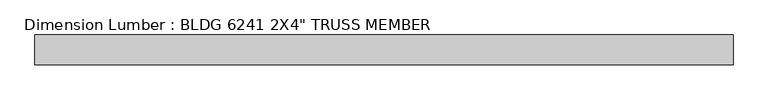
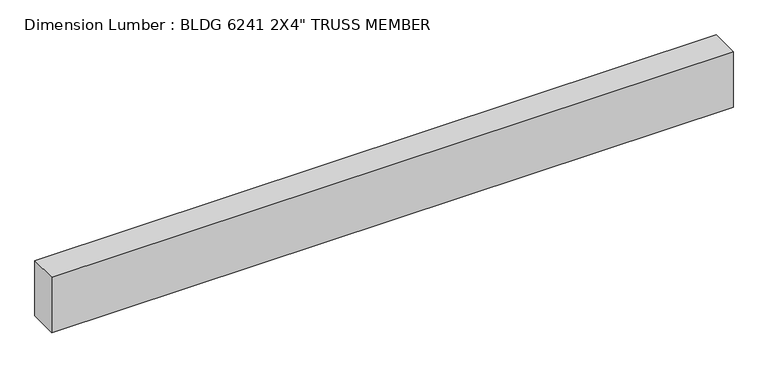
"""IFC4 building model written with IfcOpenShell, lengths in millimetres: beam geometry."""

import ifcopenshell
import ifcopenshell.guid

model = None  # the IFC model being written
_history = None  # IfcOwnerHistory: only IFC2X3 demands one
_inside = {}  # id of a spatial element -> (the spatial element, [elements in it])
_under = {}  # id of a project, library or spatial element -> (it, [spatial elements below it])
_declared = {}  # id of a project -> (the project, [libraries it declares])
_typed = {}  # id of a type object -> (the type object, [elements of that type])
_made_of = {}  # id of a material, layer set ... -> (it, [elements and type objects made of it])


def new_model(schema):
    """Start an empty IFC model of exactly this schema.

    Asked for "IFC4X3", IfcOpenShell would pick the latest addendum, in which some entities
    have other attributes; the version numbers below select the first issue.
    IFC2X3 requires an IfcOwnerHistory on every rooted entity: one is made here for all.
    """
    global model, _history
    if schema == "IFC4X3":
        model = ifcopenshell.file(schema_version=(4, 3, 0, 0))
    else:
        model = ifcopenshell.file(schema=schema)
    _inside.clear()
    _under.clear()
    _declared.clear()
    _typed.clear()
    _made_of.clear()
    _history = None
    if model.schema == "IFC2X3":
        org = make("IfcOrganization", Name="unknown")
        user = make(
            "IfcPersonAndOrganization",
            ThePerson=make("IfcPerson", FamilyName="unknown"),
            TheOrganization=org,
        )
        app = make(
            "IfcApplication",
            ApplicationDeveloper=org,
            Version="unknown",
            ApplicationFullName="unknown",
            ApplicationIdentifier="unknown",
        )
        _history = make(
            "IfcOwnerHistory",
            OwningUser=user,
            OwningApplication=app,
            ChangeAction="ADDED",
            CreationDate=0,
        )
    return model


def make(cls, **values):
    """One entity of the class cls with the attributes given. An attribute that is None is left unset."""
    return model.create_entity(
        cls, **{name: value for name, value in values.items() if value is not None}
    )


def rooted(cls, **values):
    """An entity with a GlobalId (a new one), such as an element, a storey or a relation."""
    return make(cls, GlobalId=ifcopenshell.guid.new(), OwnerHistory=_history, **values)


def si_unit(unit_type, name, prefix=None):
    """IfcSIUnit, for example si_unit("LENGTHUNIT", "METRE", prefix="MILLI")."""
    return make("IfcSIUnit", UnitType=unit_type, Prefix=prefix, Name=name)


def assignment(units):
    """IfcUnitAssignment: the units of a project."""
    return None if units is None else make("IfcUnitAssignment", Units=units)


def point(xyz):
    """IfcCartesianPoint."""
    return None if xyz is None else make("IfcCartesianPoint", Coordinates=xyz)


def direction(xyz):
    """IfcDirection."""
    return None if xyz is None else make("IfcDirection", DirectionRatios=xyz)


def frame(location, z_axis=None, x_axis=None):
    """IfcAxis2Placement3D, a coordinate frame: its origin and axes. An axis left out is left unset."""
    return make(
        "IfcAxis2Placement3D",
        Location=point(location),
        Axis=direction(z_axis),
        RefDirection=direction(x_axis),
    )


def origin():
    """The frame at (0, 0, 0) with its axes left unset."""
    return frame((0.0, 0.0, 0.0))


def place(relative_to, where):
    """IfcLocalPlacement: puts the frame where relative to a parent placement (None: the world)."""
    return make(
        "IfcLocalPlacement", PlacementRelTo=relative_to, RelativePlacement=where
    )


def context(
    kind, dimensions, precision=None, world=None, true_north=None, identifier=None
):
    """IfcGeometricRepresentationContext, for example the 3D "Model" context."""
    return make(
        "IfcGeometricRepresentationContext",
        ContextIdentifier=identifier,
        ContextType=kind,
        CoordinateSpaceDimension=dimensions,
        Precision=precision,
        WorldCoordinateSystem=world,
        TrueNorth=true_north,
    )


def project(units=None, contexts=None):
    """IfcProject with its units and contexts."""
    return rooted(
        "IfcProject",
        Name="project",
        RepresentationContexts=contexts,
        UnitsInContext=assignment(units),
    )


def spatial(cls, under=None, at=None, **own):
    """A site, building, storey or space (cls), placed at a placement, below another one or the project."""
    s = rooted(cls, ObjectPlacement=at, **own)
    if under is not None:
        _under.setdefault(under.id(), (under, []))[1].append(s)
    return s


def polyline(points):
    """IfcPolyline through the points."""
    return make("IfcPolyline", Points=[point(p) for p in points])


def outline(outer, holes=None, kind="AREA"):
    """IfcArbitraryClosedProfileDef: a profile drawn as a closed curve; with holes, ...WithVoids."""
    if holes is None:
        return make("IfcArbitraryClosedProfileDef", ProfileType=kind, OuterCurve=outer)
    return make(
        "IfcArbitraryProfileDefWithVoids",
        ProfileType=kind,
        OuterCurve=outer,
        InnerCurves=holes,
    )


def extrude(swept, where, along, depth):
    """IfcExtrudedAreaSolid: the profile swept, set in the frame where, extruded along a direction by depth."""
    return make(
        "IfcExtrudedAreaSolid",
        SweptArea=swept,
        Position=where,
        ExtrudedDirection=direction(along),
        Depth=depth,
    )


def shape(context_of_items, identifier, shape_type, items):
    """IfcShapeRepresentation: the items that make up one representation, for example the "Body"."""
    return make(
        "IfcShapeRepresentation",
        ContextOfItems=context_of_items,
        RepresentationIdentifier=identifier,
        RepresentationType=shape_type,
        Items=items,
    )


def source(mapping_origin, context_of_items, identifier, shape_type, items):
    """IfcRepresentationMap: a shape defined once, which mapped items show again and again."""
    return make(
        "IfcRepresentationMap",
        MappingOrigin=mapping_origin,
        MappedRepresentation=shape(context_of_items, identifier, shape_type, items),
    )


def transform(
    local_origin,
    x_axis=None,
    y_axis=None,
    z_axis=None,
    scale=None,
    scale2=None,
    scale3=None,
    uniform=True,
):
    """IfcCartesianTransformationOperator3D, or its non-uniform kind. x_axis, y_axis, z_axis: its Axis1, 2, 3."""
    if uniform:
        return make(
            "IfcCartesianTransformationOperator3D",
            Axis1=direction(x_axis),
            Axis2=direction(y_axis),
            LocalOrigin=point(local_origin),
            Scale=scale,
            Axis3=direction(z_axis),
        )
    return make(
        "IfcCartesianTransformationOperator3DnonUniform",
        Axis1=direction(x_axis),
        Axis2=direction(y_axis),
        LocalOrigin=point(local_origin),
        Scale=scale,
        Axis3=direction(z_axis),
        Scale2=scale2,
        Scale3=scale3,
    )


def mapped(mapping_source, mapping_target):
    """IfcMappedItem: shows the shape of a source again, moved by a transform."""
    return make(
        "IfcMappedItem", MappingSource=mapping_source, MappingTarget=mapping_target
    )


def made_of(thing, what):
    """Note that an element or type object is made of a material, layer set ...; save() writes the relation."""
    if what is not None:
        _made_of.setdefault(what.id(), (what, []))[1].append(thing)
    return thing


def element(
    cls,
    number,
    at=None,
    inside=None,
    cuts=None,
    type_object=None,
    material=None,
    context=None,
    identifier="Body",
    shape_type=None,
    held_by="IfcProductDefinitionShape",
    body=None,
    shapes=None,
    **own,
):
    """One element of the class cls, such as IfcWall. Its Tag is "e" and its number.

    at: its placement. inside: the storey or other place that contains it. cuts: it is an
    opening in that element (IfcRelVoidsElement). A single representation is given by context,
    identifier, shape_type and body (its items); several are given by shapes. held_by: the class
    of the entity that holds the representations. save() writes the other relations.
    """
    e = rooted(cls, Tag="e%d" % number, ObjectPlacement=at, **own)
    if body is not None:
        shapes = [shape(context, identifier, shape_type, body)]
    if shapes is not None:
        e.Representation = make(held_by, Representations=shapes)
    if inside is not None:
        _inside.setdefault(inside.id(), (inside, []))[1].append(e)
    if cuts is not None:
        rooted(
            "IfcRelVoidsElement", RelatingBuildingElement=cuts, RelatedOpeningElement=e
        )
    if type_object is not None:
        _typed.setdefault(type_object.id(), (type_object, []))[1].append(e)
    return made_of(e, material)


def aggregate(whole, parts):
    """IfcRelAggregates: a whole, such as a stair, and the parts it consists of."""
    return rooted("IfcRelAggregates", RelatingObject=whole, RelatedObjects=parts)


def save(model, path):
    """Write the relations noted so far, then the file.

    IfcRelAggregates (storeys below a building ...), IfcRelContainedInSpatialStructure (elements
    in a storey), IfcRelDefinesByType, IfcRelAssociatesMaterial and IfcRelDeclares: one each for
    every whole, place, type object, material and project.
    """
    for whole, parts in _under.values():
        aggregate(whole, parts)
    for where, things in _inside.values():
        rooted(
            "IfcRelContainedInSpatialStructure",
            RelatedElements=things,
            RelatingStructure=where,
        )
    for kind, things in _typed.values():
        rooted("IfcRelDefinesByType", RelatedObjects=things, RelatingType=kind)
    for what, things in _made_of.values():
        rooted("IfcRelAssociatesMaterial", RelatedObjects=things, RelatingMaterial=what)
    for by, libraries in _declared.values():
        rooted("IfcRelDeclares", RelatingContext=by, RelatedDefinitions=libraries)
    model.write(path)


def beam_a8bd1fc0(model_context):
    return source(origin(), model_context, "Body", "SweptSolid", [
        extrude(outline(polyline([(571.5, -25.4), (-609.6, -25.4), (-609.6, 25.4), (571.5, 25.4), (571.5, -25.4)])), frame((0.0, 0.0, -50.8), z_axis=(0.0, 0.0, 1.0), x_axis=(1.0, 0.0, 0.0)), (0.0, 0.0, 1.0), 101.6),
    ])


if __name__ == "__main__":
    model = new_model("IFC4")
    model_context = context("Model", 3, world=origin())
    ifc_project = project(units=[si_unit("LENGTHUNIT", "METRE", prefix="MILLI")], contexts=[model_context])
    site = spatial("IfcSite", under=ifc_project)
    building = spatial("IfcBuilding", under=site)
    placement = place(None, origin())
    beam_shape = beam_a8bd1fc0(model_context)
    element("IfcBeam", 1, ObjectType="Dimension Lumber : BLDG 6241 2X4\" TRUSS MEMBER", at=placement, inside=building, context=model_context, shape_type="MappedRepresentation", body=[
        mapped(beam_shape, transform((0.0, 0.0, 0.0), x_axis=(1.0, 0.0, 0.0), y_axis=(0.0, 1.0, 0.0), z_axis=(0.0, 0.0, 1.0))),
    ])
    save(model, "model.ifc")

# Revit data of these elements
# Type "Dimension Lumber : BLDG 6241 2X4\" TRUSS MEMBER"
#   Assembly Code = "B10"
#   A = 0.273472 SF
#   Length [instance default] = 5' - 0"
#   b = 0' - 2"
#   d = 0' - 4"
#   Structural Material [instance default] = Softwood, Lumber
# Element 1 (IfcBeam, "Dimension Lumber : BLDG 6241 2X4\" TRUSS MEMBER")
#   Materials on its faces: "Softwood, Lumber"
# Materials
#   "Softwood, Lumber": class "Wood", colour RGB 223 192 134, transparency 0, Description = "Pinus Echinata", Cost = 0
